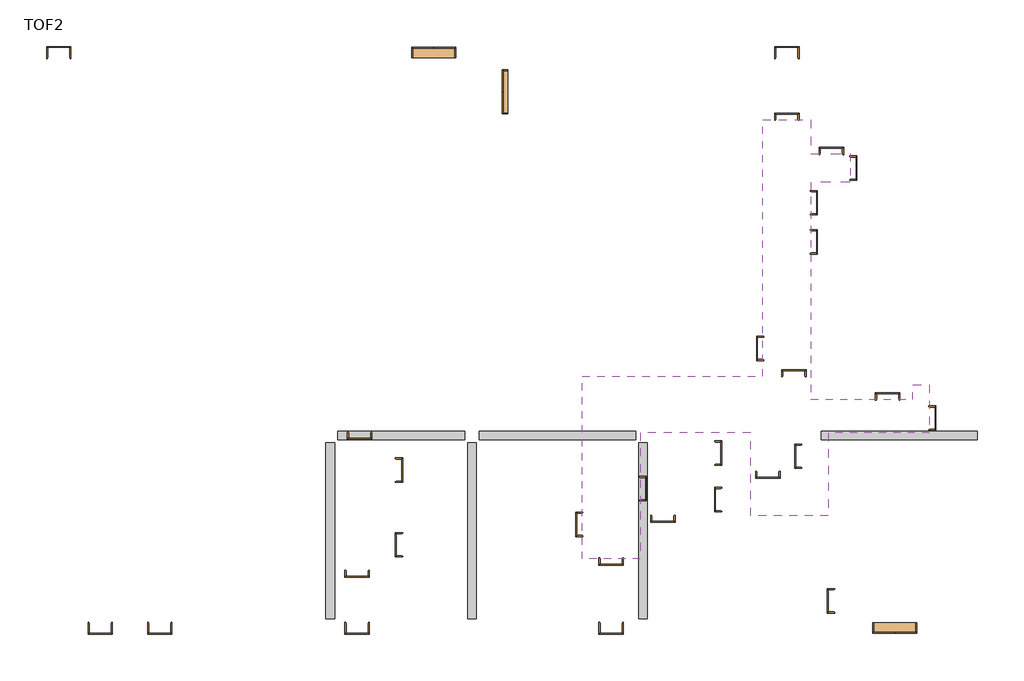
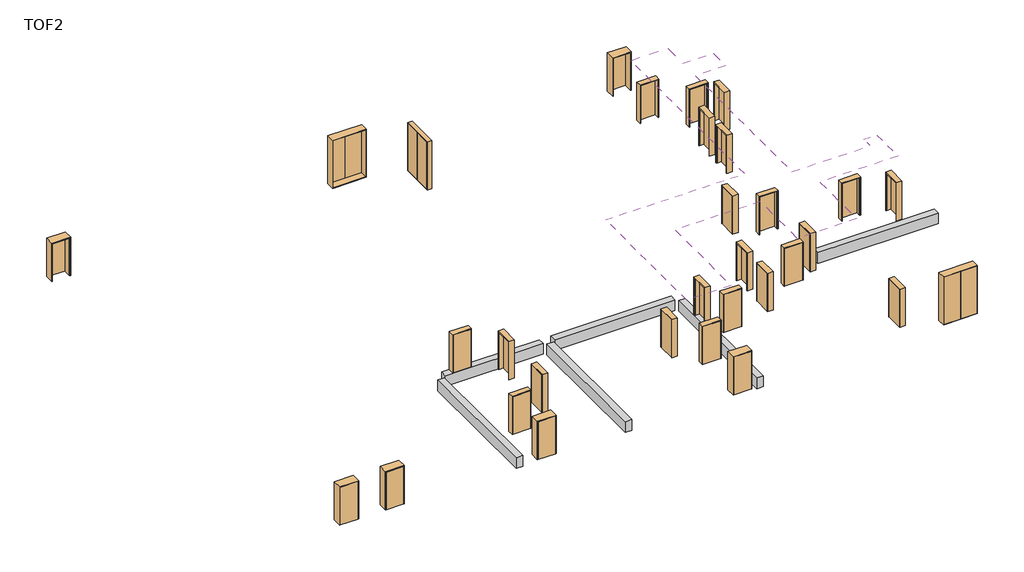
# One storey: 31 doors, 6 beams, 1 covering.
# Revit data of these elements (continued)
# Room at (44824.7, 22985.521) mm, phase "New Construction", upper level "TOC", upper offset 6500.000 mm, lower offset -1000.000 mm (continued)
#   Floor Finish Style Name = "Vinyl Tile on Screed + Matwell"
#   Base Finish Style Name = "Coved Vinyl Tile"
#   Base Finish Ref. = ""
#   Base-Base Material = "Concrete Wall\n/ Masonry Wall"
#   Base Finish-1 = ""
#   Base Finish-2 = ""
#   Base Finish-3 = "Vinyl Tile"
#   Base Finish-4 = ""
#   Wall Finish-1 = "Acrylic Emulsion Paint on Cement Plaster"
#   Wall Finish-2 = "T13 Plaster"
#   Wall Finish-3 = "Masonry Wall"
#   Wall Finish-4 = "Plastering"
#   Ceiling Finish Style Name = "Suspended Acoustic Tiled Ceiling (T-Bar)"
#   Ceiling Finish Ref. = "600x600\nT Bar"
#   Ceiling-Base Material = "Concrete Slab"
#   Ceiling Finish-1 = ""
#   Ceiling Finish-2 = ""
#   Ceiling Finish-3 = "Acoustic Tiled Ceiling System (T-Bar)"
#   Ceiling Finish-4 = ""
#   H_Room L = 2600.000 mm
#   H_Room W = 2200.000 mm
#   H_Room H or CH = 6300.000 mm
#   Floor Finish Style No = F34A-1
#   Base Finish Style No = B35A
#   Wall Finish Style No = W01B
#   Ceiling Finish Style No = C95A
# Room at (47424.7, 22284.021) mm, phase "New Construction", upper level "TOC", upper offset 6500.000 mm, lower offset -1000.000 mm
#   Comments = ""
#   Number = "105"
#   Name = "LIBRARY"
#   Floor Finish Style Name = "Vinyl Tile on Screed"
#   Floor Finish Ref. = ""
#   Floor-Base Material = "Concrete Slab"
#   Floor Finish-1 = "Screed"
#   Floor Finish-2 = ""
#   Floor Finish-3 = "Vinyl Tile"
#   Floor Finish-4 = ""
#   Base Finish Style Name = "Coved Vinyl Tile"
#   Base Finish Ref. = ""
#   Base-Base Material = "Concrete Wall\n/ Masonry Wall"
#   Base Finish-1 = ""
#   Base Finish-2 = ""
#   Base Finish-3 = "Vinyl Tile"
#   Base Finish-4 = ""
#   Wall Finish-1 = "Acrylic Emulsion Paint on Cement Plaster"
#   Wall Finish-2 = "T13 Plaster"
#   Wall Finish-3 = "Masonry Wall"
#   Wall Finish-4 = "Plastering"
#   Ceiling Finish Style Name = "Suspended Acoustic Tiled Ceiling (T-Bar)"
#   Ceiling Finish Ref. = "600x600\nT Bar"
#   Ceiling-Base Material = "Concrete Slab"
#   Ceiling Finish-1 = ""
#   Ceiling Finish-2 = ""
#   Ceiling Finish-3 = "Acoustic Tiled Ceiling System (T-Bar)"
#   Ceiling Finish-4 = ""
#   H_Room L = 4000.000 mm
#   H_Room W = 3000.000 mm
#   H_Room H or CH = 6300.000 mm
#   Floor Finish Style No = F34A
#   Base Finish Style No = B35A
#   Wall Finish Style No = W01B
#   Ceiling Finish Style No = C95A
# Room at (50025.7, 21584.021) mm, phase "New Construction", upper level "TOC", upper offset 6500.000 mm, lower offset -1000.000 mm
#   Comments = ""
#   Number = "106"
#   Name = "SHIFT SUPERVISOR/DAY SUPERVISOR"
#   Floor Finish Style Name = "Vinyl Tile on Screed"
#   Floor Finish Ref. = ""
#   Floor-Base Material = "Concrete Slab"
#   Floor Finish-1 = "Screed"
#   Floor Finish-2 = ""
#   Floor Finish-3 = "Vinyl Tile"
#   Floor Finish-4 = ""
#   Base Finish Style Name = "Coved Vinyl Tile"
#   Base Finish Ref. = ""
#   Base-Base Material = "Concrete Wall\n/ Masonry Wall"
#   Base Finish-1 = ""
#   Base Finish-2 = ""
#   Base Finish-3 = "Vinyl Tile"
#   Base Finish-4 = ""
#   Wall Finish-1 = "Acrylic Emulsion Paint on Cement Plaster"
#   Wall Finish-2 = "T13 Plaster"
#   Wall Finish-3 = "Masonry Wall"
#   Wall Finish-4 = "Plastering"
#   Ceiling Finish Style Name = "Suspended Acoustic Tiled Ceiling (T-Bar)"
#   Ceiling Finish Ref. = "600x600\nT Bar"
#   Ceiling-Base Material = "Concrete Slab"
#   Ceiling Finish-1 = ""
#   Ceiling Finish-2 = ""
#   Ceiling Finish-3 = "Acoustic Tiled Ceiling System (T-Bar)"
#   Ceiling Finish-4 = ""
#   H_Room L = 5400.000 mm
#   H_Room W = 5400.000 mm
#   H_Room H or CH = 6300.000 mm
#   Floor Finish Style No = F34A
#   Base Finish Style No = B35A
#   Wall Finish Style No = W01B
#   Ceiling Finish Style No = C95A
# Room at (25599.7, 16059.021) mm, phase "New Construction", upper level "TOC", upper offset 6500.000 mm, lower offset -1000.000 mm
#   Comments = ""
#   Number = "102"
#   Name = "RACK ROOM [F-1]"
#   Floor Finish Style Name = "Anti-Dust Epoxy Paint on Steel trowel Finish + Anti-Static Vinyl Tile on Raised Floor"
#   Floor Finish Ref. = "600x600, H=1000"
#   Floor-Base Material = "Concrete Slab"
#   Floor Finish-1 = "Steel Trowel Finish"
#   Floor Finish-2 = "Anti-Dust Paint"
#   Floor Finish-3 = "Raised Floor_Anti-Static Vinyl Tile"
#   Floor Finish-4 = ""
#   Base Finish Style Name = "Coved Vinyl Tile"
#   Base Finish Ref. = ""
#   Base-Base Material = "Concrete Wall\n/ Masonry Wall"
#   Base Finish-1 = ""
#   Base Finish-2 = ""
#   Base Finish-3 = "Vinyl Tile"
#   Base Finish-4 = ""
#   Wall Finish-1 = "Acrylic Emulsion Paint on Cement Plaster"
#   Wall Finish-2 = "T13 Plaster"
#   Wall Finish-3 = "Masonry Wall"
#   Wall Finish-4 = "Plastering"
#   Ceiling Finish Style Name = "Suspended Acoustic Tiled Ceiling (T-Bar)"
#   Ceiling Finish Ref. = "600x600\nT Bar"
#   Ceiling-Base Material = "Concrete Slab"
#   Ceiling Finish-1 = ""
#   Ceiling Finish-2 = ""
#   Ceiling Finish-3 = "Acoustic Tiled Ceiling System (T-Bar)"
#   Ceiling Finish-4 = ""
#   H_Room L = 15600.000 mm
#   H_Room W = 15300.000 mm
#   H_Room H or CH = 3000.000 mm
#   Floor Finish Style No = F91
#   Base Finish Style No = B35A
#   Wall Finish Style No = W01B
#   Ceiling Finish Style No = C95A
# Room at (40466.2, 6715.021) mm, phase "New Construction", upper level "TOC", upper offset 6500.000 mm, lower offset -1000.000 mm
#   Comments = ""
#   Number = "121"
#   Name = "LOCKER"
#   Floor Finish Style Name = "Non-Slip Unglazed Ceramic Tile on Screed"
#   Floor Finish Ref. = ""
#   Floor-Base Material = "Concrete Slab"
#   Floor Finish-1 = "Screed"
#   Floor Finish-2 = ""
#   Floor Finish-3 = "Ceramic Tile"
#   Floor Finish-4 = ""
#   Base Finish Style Name = "Coved Ceramic Tile"
#   Base Finish Ref. = ""
#   Base-Base Material = "Concrete Wall\n/ Masonry Wall"
#   Base Finish-1 = ""
#   Base Finish-2 = ""
#   Base Finish-3 = "Glazed Ceramic Tile"
#   Base Finish-4 = ""
#   Wall Finish-1 = "Glazed Ceramic Tile (<=2100) / Acrylic Emulsion Paint (>2100) on Cement Plaster"
#   Wall Finish-2 = "H=2100"
#   Ceiling Finish Style Name = "Suspended Moisture Resistant Tiled Ceiling (T-Bar)"
#   Ceiling Finish Ref. = "600x600\nT bar"
#   Ceiling-Base Material = "Concrete Slab"
#   Ceiling Finish-1 = ""
#   Ceiling Finish-2 = ""
#   Ceiling Finish-3 = "Moisture Resistant Tiled Ceiling System (T-Bar)"
#   Ceiling Finish-4 = ""
#   H_Room L = 3400.000 mm
#   H_Room W = 3000.000 mm
#   H_Room H or CH = 7300.000 mm
#   Floor Finish Style No = F31A
#   Base Finish Style No = B32
#   Wall Finish Style No = W32B-1
#   Ceiling Finish Style No = C96A
# Room at (51893.7, 10133.521) mm, phase "New Construction", upper level "TOC", upper offset 6500.000 mm, lower offset -1000.000 mm
#   Comments = ""
#   Number = "110"
#   Name = "ABLUTIONS"
#   Floor Finish Style Name = "Non-Slip Unglazed Ceramic Tile on Screed + Liquid Waterproofing"
#   Floor Finish Ref. = ""
#   Floor-Base Material = "Concrete Slab"
#   Floor Finish-1 = "Screed"
#   Floor Finish-2 = "Liquid Waterproofing"
#   Floor Finish-3 = "Ceramic Tile"
#   Floor Finish-4 = ""
#   Base Finish Style Name = "Coved Ceramic Tile"
#   Base Finish Ref. = ""
#   Base-Base Material = "Concrete Wall\n/ Masonry Wall"
#   Base Finish-1 = ""
#   Base Finish-2 = ""
#   Base Finish-3 = "Glazed Ceramic Tile"
#   Base Finish-4 = ""
#   Wall Finish-1 = "Glazed Ceramic Tile (<=2100) / Acrylic Emulsion Paint (>2100) on Cement Plaster"
#   Wall Finish-2 = "H=2100"
#   Ceiling Finish Style Name = "Suspended Moisture Resistant Tiled Ceiling (T-Bar)"
#   Ceiling Finish Ref. = "600x600\nT bar"
#   Ceiling-Base Material = "Concrete Slab"
#   Ceiling Finish-1 = ""
#   Ceiling Finish-2 = ""
#   Ceiling Finish-3 = "Moisture Resistant Tiled Ceiling System (T-Bar)"
#   Ceiling Finish-4 = ""
#   H_Room L = 3400.000 mm
#   H_Room W = 2200.000 mm
#   H_Room H or CH = 6300.000 mm
#   Floor Finish Style No = F31B
#   Base Finish Style No = B32
#   Wall Finish Style No = W32B-1
#   Ceiling Finish Style No = C96A
# Room at (8882.2, 6424.021) mm, phase "New Construction", upper level "TOC", upper offset 6500.000 mm, lower offset -1000.000 mm
#   Comments = ""
#   Number = "112"
#   Name = "ELECTRICAL ROOM(SS08) [F-1]"
#   Floor Finish Style Name = "Non-Slip Epoxy Paint on Screed"
#   Floor Finish Ref. = ""
#   Floor-Base Material = "Concrete Slab"
#   Floor Finish-1 = "Screed"
#   Floor Finish-2 = ""
#   Floor Finish-3 = "Epoxy Paint"
#   Floor Finish-4 = ""
#   Base Finish Style Name = "Epoxy Paint"
#   Base Finish Ref. = ""
#   Base-Base Material = "Concrete Wall\n/ Masonry Wall \n/ Dry Wall"
#   Base Finish-1 = ""
#   Base Finish-2 = ""
#   Base Finish-3 = "Epoxy Paint"
#   Base Finish-4 = ""
#   Wall Finish-1 = "Acrylic Emulsion Paint on Cement Plaster"
#   Wall Finish-2 = "T13 Plaster"
#   Wall Finish-3 = "Masonry Wall"
#   Wall Finish-4 = "Plastering"
#   Ceiling Finish Style Name = "Acrylic Emulsion Paint on Fair Faced Concrete"
#   Ceiling Finish Ref. = ""
#   Ceiling-Base Material = "Concrete Slab"
#   Ceiling Finish-1 = ""
#   Ceiling Finish-2 = ""
#   Ceiling Finish-3 = "Acrylic Emulsion Paint"
#   Ceiling Finish-4 = ""
#   H_Room L = 11700.000 mm
#   H_Room W = 18000.000 mm
#   H_Room H or CH = 7300.000 mm
#   Floor Finish Style No = F06B
#   Base Finish Style No = B03
#   Wall Finish Style No = W01B
#   Ceiling Finish Style No = C01
# Room at (22116.2, 4474.021) mm, phase "New Construction", upper level "TOC", upper offset 6500.000 mm, lower offset -1000.000 mm
#   Comments = ""
#   Number = "114"
#   Name = "BATTERY ROOM [F-1]"
#   Floor Finish Style Name = "Acid Resistant Ceramic Tile on Screed"
#   Floor Finish Ref. = ""
#   Floor-Base Material = "Concrete Slab"
#   Floor Finish-1 = "Screed"
#   Floor Finish-2 = ""
#   Floor Finish-3 = "Acid/Alkaline Resistant Tile"
#   Floor Finish-4 = ""
#   Base Finish Style Name = "Acid Resistant Ceramic Tile"
#   Base Finish Ref. = ""
#   Base-Base Material = "Concrete Wall\n/ Masonry Wall"
#   Base Finish-1 = ""
#   Base Finish-2 = ""
#   Base Finish-3 = "Acid/Alkaline Resistant Tile"
#   Base Finish-4 = ""
#   Wall Finish-1 = "Acid Resistant Paint on Cement Plaster"
#   Wall Finish-2 = "T13 Plaster"
#   Wall Finish-3 = "Masonry Wall"
#   Wall Finish-4 = "Plastering"
#   Ceiling Finish Style Name = "Acrylic Emulsion Paint on Fair Faced Concrete"
#   Ceiling Finish Ref. = ""
#   Ceiling-Base Material = "Concrete Slab"
#   Ceiling Finish-1 = ""
#   Ceiling Finish-2 = ""
#   Ceiling Finish-3 = "Acrylic Emulsion Paint"
#   Ceiling Finish-4 = ""
#   H_Room L = 7800.000 mm
#   H_Room W = 8300.000 mm
#   H_Room H or CH = 7300.000 mm
#   Floor Finish Style No = F32
#   Base Finish Style No = B33
#   Wall Finish Style No = W04B
#   Ceiling Finish Style No = C01
# Room at (34033.2, 4474.021) mm, phase "New Construction", upper level "TOC", upper offset 6500.000 mm, lower offset -1000.000 mm
#   Comments = ""
#   Number = "118"
#   Name = "DRIVERS LOUNGE"
#   Floor Finish Style Name = "Vinyl Tile on Screed"
#   Floor Finish Ref. = ""
#   Floor-Base Material = "Concrete Slab"
#   Floor Finish-1 = "Screed"
#   Floor Finish-2 = ""
#   Floor Finish-3 = "Vinyl Tile"
#   Floor Finish-4 = ""
#   Base Finish Style Name = "Coved Vinyl Tile"
#   Base Finish Ref. = ""
#   Base-Base Material = "Concrete Wall\n/ Masonry Wall"
#   Base Finish-1 = ""
#   Base Finish-2 = ""
#   Base Finish-3 = "Vinyl Tile"
#   Base Finish-4 = ""
#   Wall Finish-1 = "Acrylic Emulsion Paint on Cement Plaster"
#   Wall Finish-2 = "T13 Plaster"
#   Wall Finish-3 = "Masonry Wall"
#   Wall Finish-4 = "Plastering"
#   Ceiling Finish Style Name = "Suspended Acoustic Tiled Ceiling (T-Bar)"
#   Ceiling Finish Ref. = "600x600\nT Bar"
#   Ceiling-Base Material = "Concrete Slab"
#   Ceiling Finish-1 = ""
#   Ceiling Finish-2 = ""
#   Ceiling Finish-3 = "Acoustic Tiled Ceiling System (T-Bar)"
#   Ceiling Finish-4 = ""
#   H_Room L = 7800.000 mm
#   H_Room W = 4500.000 mm
#   H_Room H or CH = 6300.000 mm
#   Floor Finish Style No = F34A
#   Base Finish Style No = B35A
#   Wall Finish Style No = W01B
#   Ceiling Finish Style No = C95A
# Room at (41074.7, 2772.521) mm, phase "New Construction", upper level "TOC", upper offset 6500.000 mm, lower offset -1000.000 mm
#   Comments = ""
#   Number = "122"
#   Name = "TOILETS"
#   Floor Finish Style Name = "Non-Slip Unglazed Ceramic Tile on Screed + Liquid Waterproofing"
#   Floor Finish Ref. = ""
#   Floor-Base Material = "Concrete Slab"
#   Floor Finish-1 = "Screed"
#   Floor Finish-2 = "Liquid Waterproofing"
#   Floor Finish-3 = "Ceramic Tile"
#   Floor Finish-4 = ""
#   Base Finish Style Name = "Coved Ceramic Tile"
#   Base Finish Ref. = ""
#   Base-Base Material = "Concrete Wall\n/ Masonry Wall"
#   Base Finish-1 = ""
#   Base Finish-2 = ""
#   Base Finish-3 = "Glazed Ceramic Tile"
#   Base Finish-4 = ""
#   Wall Finish-1 = "Glazed Ceramic Tile (<=2100) / Acrylic Emulsion Paint (>2100) on Cement Plaster"
#   Wall Finish-2 = "H=2100"
#   Ceiling Finish Style Name = "Suspended Moisture Resistant Tiled Ceiling (T-Bar)"
#   Ceiling Finish Ref. = "600x600\nT bar"
#   Ceiling-Base Material = "Concrete Slab"
#   Ceiling Finish-1 = ""
#   Ceiling Finish-2 = ""
#   Ceiling Finish-3 = "Moisture Resistant Tiled Ceiling System (T-Bar)"
#   Ceiling Finish-4 = ""
#   H_Room L = 4400.000 mm
#   H_Room W = 4300.000 mm
#   H_Room H or CH = 7300.000 mm
#   Floor Finish Style No = F31B
#   Base Finish Style No = B32
#   Wall Finish Style No = W32B-1
#   Ceiling Finish Style No = C96A
# Room at (37624.7, 1897.521) mm, phase "New Construction", upper level "TOC", upper offset 6500.000 mm, lower offset -1000.000 mm
#   Comments = ""
#   Number = "119"
#   Name = "AIR LOCK"
#   Floor Finish Style Name = "Vinyl Tile on Screed + Matwell"
#   Base Finish Style Name = "Coved Vinyl Tile"
#   Base Finish Ref. = ""
#   Base-Base Material = "Concrete Wall\n/ Masonry Wall"
#   Base Finish-1 = ""
#   Base Finish-2 = ""
#   Base Finish-3 = "Vinyl Tile"
#   Base Finish-4 = ""
#   Wall Finish-1 = "Acrylic Emulsion Paint on Cement Plaster"
#   Wall Finish-2 = "T13 Plaster"
#   Wall Finish-3 = "Masonry Wall"
#   Wall Finish-4 = "Plastering"
#   Ceiling Finish Style Name = "Suspended Acoustic Tiled Ceiling (T-Bar)"
#   Ceiling Finish Ref. = "600x600\nT Bar"
#   Ceiling-Base Material = "Concrete Slab"
#   Ceiling Finish-1 = ""
#   Ceiling Finish-2 = ""
#   Ceiling Finish-3 = "Acoustic Tiled Ceiling System (T-Bar)"
#   Ceiling Finish-4 = ""
#   H_Room L = 2700.000 mm
#   H_Room W = 2600.000 mm
#   H_Room H or CH = 6300.000 mm
#   Floor Finish Style No = F34A-1
#   Base Finish Style No = B35A
#   Wall Finish Style No = W01B
#   Ceiling Finish Style No = C95A
# Room at (44924.7, 2772.521) mm, phase "New Construction", upper level "TOC", upper offset 6500.000 mm, lower offset -1000.000 mm
#   Comments = ""
#   Number = "124"
#   Name = "STORE"
#   Floor Finish Style Name = "Vinyl Tile on Screed"
#   Floor Finish Ref. = ""
#   Floor-Base Material = "Concrete Slab"
#   Floor Finish-1 = "Screed"
#   Floor Finish-2 = ""
#   Floor Finish-3 = "Vinyl Tile"
#   Floor Finish-4 = ""
#   Base Finish Style Name = "Coved Vinyl Tile"
#   Base Finish Ref. = ""
#   Base-Base Material = "Concrete Wall\n/ Masonry Wall"
#   Base Finish-1 = ""
#   Base Finish-2 = ""
#   Base Finish-3 = "Vinyl Tile"
#   Base Finish-4 = ""
#   Wall Finish-1 = "Acrylic Emulsion Paint on Cement Plaster"
#   Wall Finish-2 = "T13 Plaster"
#   Wall Finish-3 = "Masonry Wall"
#   Wall Finish-4 = "Plastering"
#   Ceiling Finish Style Name = "Suspended Acoustic Tiled Ceiling (T-Bar)"
#   Ceiling Finish Ref. = "600x600\nT Bar"
#   Ceiling-Base Material = "Concrete Slab"
#   Ceiling Finish-1 = ""
#   Ceiling Finish-2 = ""
#   Ceiling Finish-3 = "Acoustic Tiled Ceiling System (T-Bar)"
#   Ceiling Finish-4 = ""
#   H_Room L = 4400.000 mm
#   H_Room W = 3400.000 mm
#   H_Room H or CH = 7300.000 mm
#   Floor Finish Style No = F34A
#   Base Finish Style No = B35A
#   Wall Finish Style No = W01B
#   Ceiling Finish Style No = C95A
# Room at (49817.2, 4474.021) mm, phase "New Construction", upper level "TOC", upper offset 6500.000 mm, lower offset -1000.000 mm
#   Comments = ""
#   Number = "125"
#   Name = "MAINTENANCE WORKSHOP [F-1]"
#   Floor Finish Style Name = "Non-Slip Epoxy Paint on Steel Trowel Finish"
#   Floor Finish Ref. = ""
#   Floor-Base Material = "Concrete Slab"
#   Floor Finish-1 = "Steel Trowel Finish"
#   Floor Finish-2 = ""
#   Floor Finish-3 = "Epoxy Paint"
#   Floor Finish-4 = ""
#   Base Finish Style Name = "Epoxy Paint"
#   Base Finish Ref. = ""
#   Base-Base Material = "Concrete Wall\n/ Masonry Wall \n/ Dry Wall"
#   Base Finish-1 = ""
#   Base Finish-2 = ""
#   Base Finish-3 = "Epoxy Paint"
#   Base Finish-4 = ""
#   Wall Finish-1 = "Acrylic Emulsion Paint on Cement Plaster"
#   Wall Finish-2 = "T13 Plaster"
#   Wall Finish-3 = "Masonry Wall"
#   Wall Finish-4 = "Plastering"
#   Ceiling Finish Style Name = "Acrylic Emulsion Paint on Fair Faced Concrete"
#   Ceiling Finish Ref. = ""
#   Ceiling-Base Material = "Concrete Slab"
#   Ceiling Finish-1 = ""
#   Ceiling Finish-2 = ""
#   Ceiling Finish-3 = "Acrylic Emulsion Paint"
#   Ceiling Finish-4 = ""
#   H_Room L = 7800.000 mm
#   H_Room W = 7700.000 mm
#   H_Room H or CH = 7300.000 mm
#   Floor Finish Style No = F06A
#   Base Finish Style No = B03
#   Wall Finish Style No = W01B
#   Ceiling Finish Style No = C01
# Room at (43973.125, 9512.388) mm, phase "New Construction", upper level "TOC", upper offset 6500.000 mm, lower offset -1000.000 mm
#   Comments = ""
#   Number = "120"
#   Name = "CORRIDOR"
#   Floor Finish Style Name = "Vinyl Tile on Screed"
#   Floor Finish Ref. = ""
#   Floor-Base Material = "Concrete Slab"
#   Floor Finish-1 = "Screed"
#   Floor Finish-2 = ""
#   Floor Finish-3 = "Vinyl Tile"
#   Floor Finish-4 = ""
#   Base Finish Style Name = "Coved Vinyl Tile"
#   Base Finish Ref. = ""
#   Base-Base Material = "Concrete Wall\n/ Masonry Wall"
#   Base Finish-1 = ""
#   Base Finish-2 = ""
#   Base Finish-3 = "Vinyl Tile"
#   Base Finish-4 = ""
#   Wall Finish-1 = "Acrylic Emulsion Paint on Cement Plaster"
#   Wall Finish-2 = "T13 Plaster"
#   Wall Finish-3 = "Masonry Wall"
#   Wall Finish-4 = "Plastering"
#   Ceiling Finish Style Name = "Suspended Acoustic Tiled Ceiling (T-Bar)"
#   Ceiling Finish Ref. = "600x600\nT Bar"
#   Ceiling-Base Material = "Concrete Slab"
#   Ceiling Finish-1 = ""
#   Ceiling Finish-2 = ""
#   Ceiling Finish-3 = "Acoustic Tiled Ceiling System (T-Bar)"
#   Ceiling Finish-4 = ""
#   H_Room L = 7700.000 mm
#   H_Room W = 14400.000 mm
#   H_Room H or CH = 3600.000 mm
#   Floor Finish Style No = F34A
#   Base Finish Style No = B35A
#   Wall Finish Style No = W01B
#   Ceiling Finish Style No = C95A
# Room at (44840.524, 5924.958) mm, phase "New Construction", upper level "TOC", upper offset 6500.000 mm, lower offset 0.000 mm
#   Comments = ""
#   Number = "123"
#   Name = "STORE"
#   Floor Finish Style Name = "Vinyl Tile on Screed"
#   Floor Finish Ref. = ""
#   Floor-Base Material = "Concrete Slab"
#   Floor Finish-1 = "Screed"
#   Floor Finish-2 = ""
#   Floor Finish-3 = "Vinyl Tile"
#   Floor Finish-4 = ""
#   Base Finish Style Name = "Coved Vinyl Tile"
#   Base Finish Ref. = ""
#   Base-Base Material = "Concrete Wall\n/ Masonry Wall"
#   Base Finish-1 = ""
#   Base Finish-2 = ""
#   Base Finish-3 = "Vinyl Tile"
#   Base Finish-4 = ""
#   Wall Finish-1 = "Acrylic Emulsion Paint on Cement Plaster"
#   Wall Finish-2 = "T13 Plaster"
#   Wall Finish-3 = "Masonry Wall"
#   Wall Finish-4 = "Plastering"
#   Ceiling Finish Style Name = "Suspended Acoustic Tiled Ceiling (T-Bar)"
#   Ceiling Finish Ref. = "600x600\nT Bar"
#   Ceiling-Base Material = "Concrete Slab"
#   Ceiling Finish-1 = ""
#   Ceiling Finish-2 = ""
#   Ceiling Finish-3 = "Acoustic Tiled Ceiling System (T-Bar)"
#   Ceiling Finish-4 = ""
#   H_Room L = 1800.000 mm
#   H_Room W = 3400.000 mm
#   H_Room H or CH = 3700.000 mm
#   Floor Finish Style No = F34A
#   Base Finish Style No = B35A
#   Wall Finish Style No = W01B
#   Ceiling Finish Style No = C95A
# Room at (45068.625, 15370.439) mm, phase "New Construction", upper level "TOC", upper offset 6500.000 mm, lower offset 0.000 mm
#   Comments = ""
#   Number = "107"
#   Name = "CORRIDOR"
#   Floor Finish Style Name = "Vinyl Tile on Screed"
#   Floor Finish Ref. = ""
#   Floor-Base Material = "Concrete Slab"
#   Floor Finish-1 = "Screed"
#   Floor Finish-2 = ""
#   Floor Finish-3 = "Vinyl Tile"
#   Floor Finish-4 = ""
#   Base Finish Style Name = "Coved Vinyl Tile"
#   Base Finish Ref. = ""
#   Base-Base Material = "Concrete Wall\n/ Masonry Wall"
#   Base Finish-1 = ""
#   Base Finish-2 = ""
#   Base Finish-3 = "Vinyl Tile"
#   Base Finish-4 = ""
#   Wall Finish-1 = "Acrylic Emulsion Paint on Cement Plaster"
#   Wall Finish-2 = "T13 Plaster"
#   Wall Finish-3 = "Masonry Wall"
#   Wall Finish-4 = "Plastering"
#   Ceiling Finish Style Name = "Suspended Acoustic Tiled Ceiling (T-Bar)"
#   Ceiling Finish Ref. = "600x600\nT Bar"
#   Ceiling-Base Material = "Concrete Slab"
#   Ceiling Finish-1 = ""
#   Ceiling Finish-2 = ""
#   Ceiling Finish-3 = "Acoustic Tiled Ceiling System (T-Bar)"
#   Ceiling Finish-4 = ""
#   H_Room L = 10500.000 mm
#   H_Room W = 3800.000 mm
#   H_Room H or CH = 3700.000 mm
#   Floor Finish Style No = F34A
#   Base Finish Style No = B35A
#   Wall Finish Style No = W01B
#   Ceiling Finish Style No = C95A
